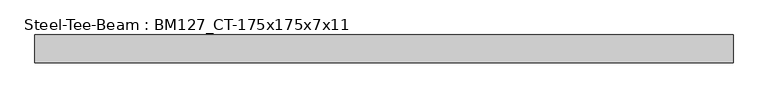
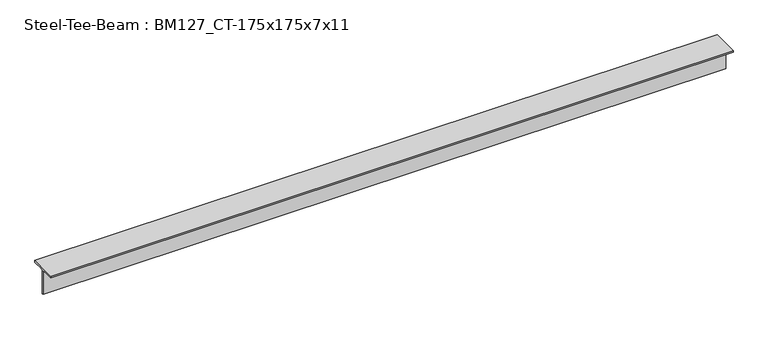
"""IFC4 building model written with IfcOpenShell, lengths in millimetres: beam geometry, Steel-Tee-Beam : BM127_CT-175x175x7x11."""

from ifc_helpers import new_model, si_unit, point, frame, frame_2d, origin, place, context, project, spatial, polyline, circle_curve, trimmed, segment, composite_curve, outline, extrude, source, transform, mapped, element, save


def steel_tee_beam_bm127_ct_175x175x7x11_b3259496(model_context):
    return source(origin(), model_context, "Body", "SweptSolid", [
        extrude(outline(composite_curve([segment(polyline([(87.5, 87.5), (87.5, 76.5), (17.5, 76.5)]), True, "CONTINUOUS"), segment(trimmed(circle_curve(frame_2d((17.5, 62.5)), 14.0), [point((17.5, 76.5))], [point((3.5, 62.5))], True, "CARTESIAN"), True, "CONTINUOUS"), segment(polyline([(3.5, 62.5), (3.5, -87.5), (-3.5, -87.5), (-3.5, 62.5)]), True, "CONTINUOUS"), segment(trimmed(circle_curve(frame_2d((-17.5, 62.5)), 14.0), [point((-3.5, 62.5))], [point((-17.5, 76.5))], True, "CARTESIAN"), True, "CONTINUOUS"), segment(polyline([(-17.5, 76.5), (-87.5, 76.5), (-87.5, 87.5), (87.5, 87.5)]), True, "CONTINUOUS")], self_intersect=False)), frame((-2195.6471805, 0.0, 0.0), z_axis=(1.0, 0.0, 0.0), x_axis=(0.0, 1.0, 0.0)), (0.0, 0.0, 1.0), 4380.4779119),
    ])


if __name__ == "__main__":
    model = new_model("IFC4")
    model_context = context("Model", 3, world=origin())
    ifc_project = project(units=[si_unit("LENGTHUNIT", "METRE", prefix="MILLI")], contexts=[model_context])
    site = spatial("IfcSite", under=ifc_project)
    building = spatial("IfcBuilding", under=site)
    placement = place(None, origin())
    steel_tee_beam_bm127_ct_175x175x7x11_shape = steel_tee_beam_bm127_ct_175x175x7x11_b3259496(model_context)
    element("IfcBeam", 1, ObjectType="Steel-Tee-Beam : BM127_CT-175x175x7x11", at=placement, inside=building, context=model_context, shape_type="MappedRepresentation", body=[
        mapped(steel_tee_beam_bm127_ct_175x175x7x11_shape, transform((0.0, 0.0, 0.0), x_axis=(1.0, 0.0, 0.0), y_axis=(0.0, 1.0, 0.0), z_axis=(0.0, 0.0, 1.0))),
    ])
    save(model, "model.ifc")

# Revit data of these elements
# Type "Steel-Tee-Beam : BM127_CT-175x175x7x11"
#   Surface Area = 0.00 m²/m
#   Section Area = 31.57 cm²
#   Mass per Unit Length = 24.80 kg/m
#   Length [instance default] = 1524 mm
#   bf = 175 mm
#   d = 175 mm
#   k = 25 mm
#   kr = 14 mm
#   tf = 11 mm
#   tw = 7 mm
#   hec_material4 [instance default] = none
#   hec_material3 [instance default] = none
#   hec_material2 [instance default] = none
#   hec_material1 [instance default] = none
#   Structural Material [instance default] = Steel, 45-345
#   Assembly Code = ""
# Element 1 (IfcBeam, "Steel-Tee-Beam : BM127_CT-175x175x7x11")
#   hec_material3 = F01AC000-00002_Building/Shelter Fire Proofing Work_Intumescent Coating Type_1 hr. rating (UL 1709))
#   hec_material2 = S01AA010-00002_Main Steel Structure Fabrication Work_Shelter/Building_Steel Painting/Coating_for Fireproofed Steel Surface, Surface Preparation & Primer Coat
#   hec_material1 = S03AA029-00001_Main Steel Structure Erection Work_Shelter/Building_Light Steel
#   Structural Material = S01AA003-00001_Main Steel Structure Fabrication Work_Shelter/Building_Light Steel - Standard
#   Materials on its faces: "S01AA003-00001_Main Steel Structure Fabrication Work_Shelter/Building_Light Steel - Standard"
# Materials
#   "Steel, 45-345": class "Metal", colour RGB 189 187 185, transparency 0, Description = "Steel 345 MPa", Cost = 0
#   "S01AA003-00001_Main Steel Structure Fabrication Work_Shelter/Building_Light Steel - Standard": class "Metal", colour RGB 120 120 120, transparency 0, Comments = "(30KG/M>Weight)", Description = "Structural steel 50ksi", W00) Work Master Code = "S01AA003-00001", W01) Work Master_Lv1 = "Main Steel Structure Fabrication Work", W02) Work Master_Lv2 = "Shelter/Building", W03) Work Master_Spec.1 = "Light Steel - Standard (30KG/M>Weight)", Cost = 0
#   "F01AC000-00002_Building/Shelter Fire Proofing Work_Intumescent Coating Type_1 hr. rating (UL 1709))": class "Metal", colour RGB 255 128 128, transparency 0, Description = "Paint finished steel", W00) Work Master Code = "F01AC000-00002", W01) Work Master_Lv1 = "Building/Shelter Fire Proofing Work", W02) Work Master_Lv2 = "Intumescent Coating Type", W03) Work Master_Spec.1 = "1 hr. rating (UL 1709)", Cost = 0
#   "S01AA010-00002_Main Steel Structure Fabrication Work_Shelter/Building_Steel Painting/Coating_for Fireproofed Steel Surface, Surface Preparation & Primer Coat": class "Metal", colour RGB 120 120 120, transparency 0, Description = "Paint finished steel", W00) Work Master Code = "SS01AA010-00002", W01) Work Master_Lv1 = "Main Steel Structure Fabrication Work", W02) Work Master_Lv2 = "Shelter/Building", W03) Work Master_Spec.1 = "Steel Painting/Coating", W04) Work Master_Spec.2 = "for Fireproofed Steel Surface, Surface Preparation & Primer Coat", Cost = 0
#   "S03AA029-00001_Main Steel Structure Erection Work_Shelter/Building_Light Steel": class "Metal", colour RGB 120 120 120, transparency 0, Comments = "(30KG/M>Weight)", Description = "Structural steel 50ksi", W00) Work Master Code = "S03AA029-00001", W01) Work Master_Lv1 = "Main Steel Structure Erection Work", W02) Work Master_Lv2 = "Shelter/Building", W03) Work Master_Spec.1 = "Light Steel (30KG/M>Weight)", Cost = 0
